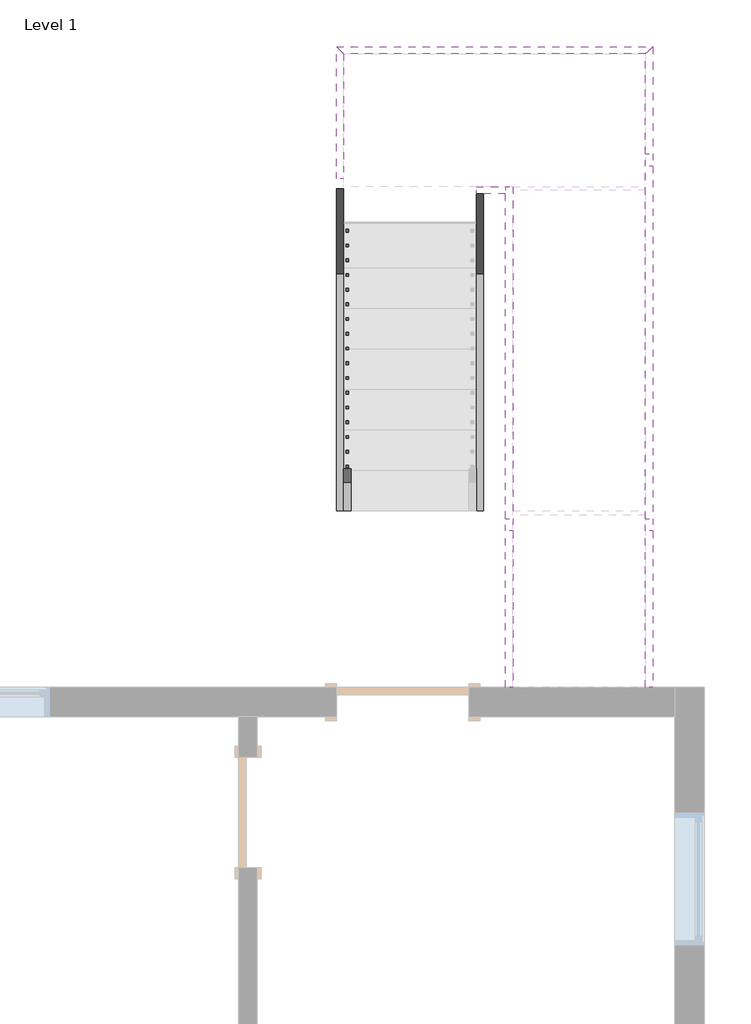
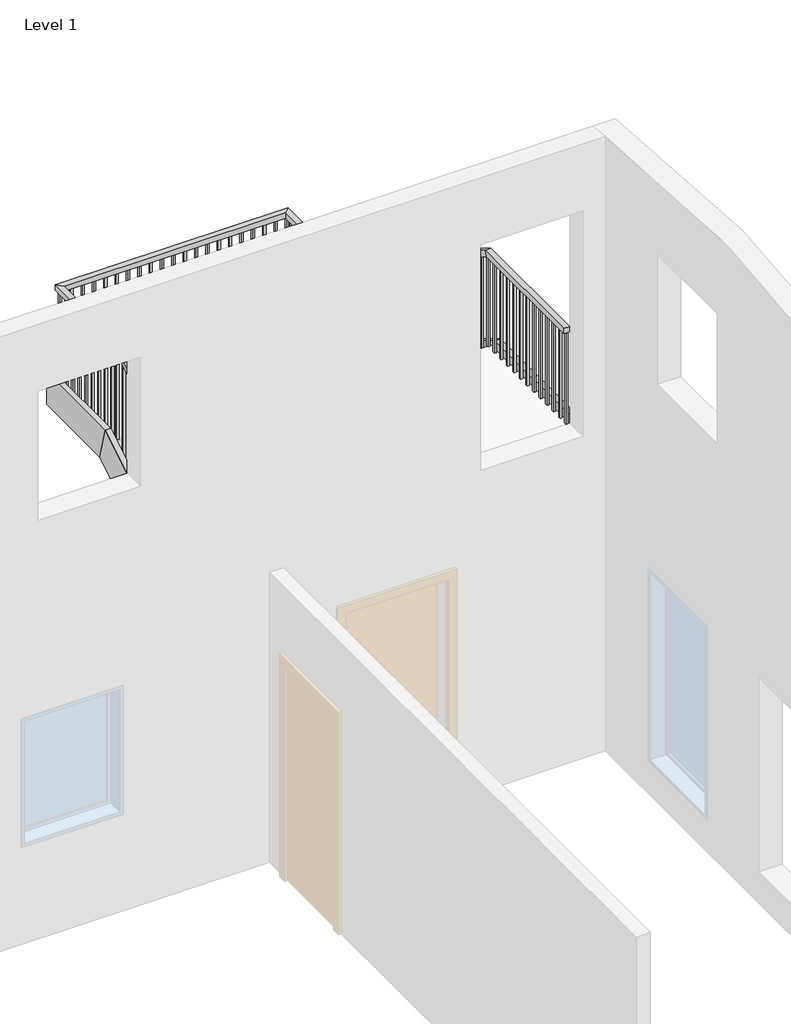
# One storey, part 3 of 3: 10 members, 1 railing.
"""IFC4 building model written with IfcOpenShell, lengths in millimetres."""

from ifc_helpers import new_model, si_unit, frame, origin, place, context, project, spatial, polyline, outline, extrude, faceted_brep, element, save

model = new_model("IFC4")

# Units and contexts
model_context = context("Model", 3, world=origin())
ifc_project = project(units=[si_unit("LENGTHUNIT", "METRE", prefix="MILLI")], contexts=[model_context])

# Site, building, storey
site = spatial("IfcSite", under=ifc_project)
building = spatial("IfcBuilding", under=site)
storey = spatial("IfcBuildingStorey", under=building, Name="Level 1", Elevation=0.0)

# Members
placement = place(None, origin())
element("IfcMember", 1, ObjectType="Stringer - 2\" Width", at=placement, inside=storey, context=model_context, shape_type="SweptSolid", body=[
    extrude(outline(polyline([(14886.0483822, 0.0), (14886.0483822, 212.114512), (17176.3894375, 1600.2), (17261.543894, 1295.4), (15124.133894, 0.0), (14886.0483822, 0.0)])), frame((14862.3123343, 0.0, 0.0), z_axis=(1.0, 0.0, 0.0), x_axis=(0.0, 1.0, 0.0)), (0.0, 0.0, 1.0), 50.8),
])
element("IfcMember", 2, ObjectType="Stringer - 2\" Width", at=placement, inside=storey, context=model_context, shape_type="SweptSolid", body=[
    extrude(outline(polyline([(14886.0483822, 0.0), (14886.0483822, 212.114512), (17070.4483822, 1535.9932998), (17070.4483822, 1179.5845383), (15124.133894, 0.0), (14886.0483822, 0.0)])), frame((15827.5123343, 0.0, 0.0), z_axis=(1.0, 0.0, 0.0), x_axis=(0.0, 1.0, 0.0)), (0.0, 0.0, 1.0), 50.8),
])
element("IfcMember", 3, ObjectType="Stringer - 2\" Width", at=placement, inside=storey, context=model_context, shape_type="SweptSolid", body=[
    extrude(outline(polyline([(17345.507327, 1600.2), (17260.3528705, 1295.4), (14745.7528705, 2819.4), (14830.907327, 3124.2), (17345.507327, 1600.2)])), frame((16995.9123343, 0.0, 0.0), z_axis=(1.0, 0.0, 0.0), x_axis=(0.0, 1.0, 0.0)), (0.0, 0.0, 1.0), 50.8),
])
element("IfcMember", 4, ObjectType="Stringer - 2\" Width", at=placement, inside=storey, context=model_context, shape_type="SweptSolid", body=[
    extrude(outline(polyline([(17121.2483822, 1736.114512), (17121.2483822, 1379.7057504), (14745.7528705, 2819.4), (14830.907327, 3124.2), (17121.2483822, 1736.114512)])), frame((16030.7123343, 0.0, 0.0), z_axis=(1.0, 0.0, 0.0), x_axis=(0.0, 1.0, 0.0)), (0.0, 0.0, 1.0), 50.8),
])
element("IfcMember", 5, ObjectType="Stringer - 2\" Width", at=placement, inside=storey, context=model_context, shape_type="Brep", body=[
    faceted_brep([(16995.9123343, 17345.507327, 1600.2), (17046.7123343, 17345.507327, 1600.2), (17046.7123343, 18086.4483822, 1600.2), (16995.9123343, 18035.6483822, 1600.2), (16995.9123343, 17260.3528705, 1295.4), (16995.9123343, 18035.6483822, 1295.4), (17046.7123343, 17260.3528705, 1295.4), (17046.7123343, 18086.4483822, 1295.4)], [[[0, 1, 2, 3]], [[4, 0, 3, 5]], [[6, 4, 5, 7]], [[1, 6, 7, 2]], [[1, 0, 4, 6]], [[2, 7, 5, 3]]]),
])
element("IfcMember", 6, ObjectType="Stringer - 2\" Width", at=placement, inside=storey, context=model_context, shape_type="SweptSolid", body=[
    extrude(outline(polyline([(17046.7123343, 18086.4483822), (16995.9123343, 18035.6483822), (14913.1123343, 18035.6483822), (14862.3123343, 18086.4483822), (17046.7123343, 18086.4483822)])), frame((0.0, 0.0, 1295.4), z_axis=(0.0, 0.0, 1.0), x_axis=(1.0, 0.0, 0.0)), (0.0, 0.0, 1.0), 304.8),
])
element("IfcMember", 7, ObjectType="Stringer - 2\" Width", at=placement, inside=storey, context=model_context, shape_type="Brep", body=[
    faceted_brep([(14913.1123343, 18035.6483822, 1600.2), (14862.3123343, 18086.4483822, 1600.2), (14862.3123343, 17176.3894375, 1600.2), (14913.1123343, 17176.3894375, 1600.2), (14913.1123343, 18035.6483822, 1295.4), (14913.1123343, 17261.543894, 1295.4), (14862.3123343, 18086.4483822, 1295.4), (14862.3123343, 17261.543894, 1295.4)], [[[0, 1, 2, 3]], [[4, 0, 3, 5]], [[6, 4, 5, 7]], [[1, 6, 7, 2]], [[1, 0, 4, 6]], [[2, 7, 5, 3]]]),
])
element("IfcMember", 8, ObjectType="Stringer - 2\" Width", at=placement, inside=storey, context=model_context, shape_type="SweptSolid", body=[
    extrude(outline(polyline([(15827.5123343, 17070.4483822), (15827.5123343, 17121.2483822), (16030.7123343, 17121.2483822), (16030.7123343, 17070.4483822), (15827.5123343, 17070.4483822)])), frame((0.0, 0.0, 1295.4), z_axis=(0.0, 0.0, 1.0), x_axis=(1.0, 0.0, 0.0)), (0.0, 0.0, 1.0), 304.8),
])
element("IfcMember", 9, ObjectType="Stringer - 2\" Width", at=placement, inside=storey, context=model_context, shape_type="SweptSolid", body=[
    extrude(outline(polyline([(13666.8483822, 2819.4), (13666.8483822, 3124.2), (14830.907327, 3124.2), (14745.7528705, 2819.4), (13666.8483822, 2819.4)])), frame((16995.9123343, 0.0, 0.0), z_axis=(1.0, 0.0, 0.0), x_axis=(0.0, 1.0, 0.0)), (0.0, 0.0, 1.0), 50.8),
])
element("IfcMember", 10, ObjectType="Stringer - 2\" Width", at=placement, inside=storey, context=model_context, shape_type="SweptSolid", body=[
    extrude(outline(polyline([(14830.907327, 3124.2), (14745.7528705, 2819.4), (13666.8483822, 2819.4), (13666.8483822, 3124.2), (14830.907327, 3124.2)])), frame((16030.7123343, 0.0, 0.0), z_axis=(1.0, 0.0, 0.0), x_axis=(0.0, 1.0, 0.0)), (0.0, 0.0, 1.0), 50.8),
])

# Railing
element("IfcRailing", 11, ObjectType="Handrail - Rectangular", at=placement, inside=storey, context=model_context, shape_type="SolidModel", body=[
    faceted_brep([(16995.9123343, 13666.8483822, 3962.4), (16945.1123343, 13666.8483822, 3962.4), (16945.1123343, 13666.8483822, 3911.6), (16995.9123343, 13666.8483822, 3911.6), (16995.9123343, 14871.8559728, 3911.6), (16995.9123343, 14886.0483822, 3962.4), (16945.1123343, 14871.8559728, 3911.6), (16945.1123343, 14886.0483822, 3962.4), (16995.9123343, 17094.918655, 2564.2892835), (16995.9123343, 17121.2483822, 2607.7333333), (16945.1123343, 17094.918655, 2564.2892835), (16945.1123343, 17121.2483822, 2607.7333333), (16995.9123343, 17386.4559728, 2387.6), (16995.9123343, 17400.6483822, 2438.4), (16945.1123343, 17386.4559728, 2387.6), (16945.1123343, 17400.6483822, 2438.4), (14913.1123343, 18035.6483822, 2387.6), (14913.1123343, 18035.6483822, 2438.4), (16995.9123343, 18035.6483822, 2438.4), (16995.9123343, 18035.6483822, 2387.6), (14963.9123343, 17984.8483822, 2387.6), (16945.1123343, 17984.8483822, 2387.6), (14963.9123343, 17984.8483822, 2438.4), (16945.1123343, 17984.8483822, 2438.4), (14913.1123343, 17135.4407916, 2387.6), (14913.1123343, 17121.2483822, 2438.4), (14963.9123343, 17135.4407916, 2387.6), (14963.9123343, 17121.2483822, 2438.4), (14913.1123343, 14886.0483822, 1083.7333333), (14913.1123343, 14886.0483822, 1024.3318731), (14963.9123343, 14886.0483822, 1024.3318731), (14963.9123343, 14886.0483822, 1083.7333333)], [[[0, 1, 2, 3]], [[4, 5, 0, 3]], [[6, 4, 3, 2]], [[7, 6, 2, 1]], [[5, 7, 1, 0]], [[8, 9, 5, 4]], [[10, 8, 4, 6]], [[11, 10, 6, 7]], [[9, 11, 7, 5]], [[12, 13, 9, 8]], [[14, 12, 8, 10]], [[15, 14, 10, 11]], [[13, 15, 11, 9]], [[16, 17, 18, 19]], [[20, 16, 19, 21]], [[22, 20, 21, 23]], [[17, 22, 23, 18]], [[24, 25, 17, 16]], [[26, 24, 16, 20]], [[27, 26, 20, 22]], [[25, 27, 22, 17]], [[28, 29, 30, 31]], [[29, 28, 25, 24]], [[30, 29, 24, 26]], [[31, 30, 26, 27]], [[28, 31, 27, 25]], [[19, 18, 13, 12]], [[21, 19, 12, 14]], [[23, 21, 14, 15]], [[18, 23, 15, 13]]]),
    extrude(outline(polyline([(14978.1233822, 1080.1349034), (14997.1733822, 1091.6803579), (14997.1733822, 169.3333333), (14978.1233822, 169.3333333), (14978.1233822, 1080.1349034)])), frame((14928.9873343, 0.0, 0.0), z_axis=(1.0, 0.0, 0.0), x_axis=(0.0, 1.0, 0.0)), (0.0, 0.0, 1.0), 19.05),
    extrude(outline(polyline([(15079.7233822, 1141.710661), (15098.7733822, 1153.2561155), (15098.7733822, 169.3333333), (15079.7233822, 169.3333333), (15079.7233822, 1141.710661)])), frame((14928.9873343, 0.0, 0.0), z_axis=(1.0, 0.0, 0.0), x_axis=(0.0, 1.0, 0.0)), (0.0, 0.0, 1.0), 19.05),
    extrude(outline(polyline([(15181.3233822, 1203.2864185), (15200.3733822, 1214.8318731), (15200.3733822, 338.6666667), (15181.3233822, 338.6666667), (15181.3233822, 1203.2864185)])), frame((14928.9873343, 0.0, 0.0), z_axis=(1.0, 0.0, 0.0), x_axis=(0.0, 1.0, 0.0)), (0.0, 0.0, 1.0), 19.05),
    extrude(outline(polyline([(15282.9233822, 1264.8621761), (15301.9733822, 1276.4076307), (15301.9733822, 338.6666667), (15282.9233822, 338.6666667), (15282.9233822, 1264.8621761)])), frame((14928.9873343, 0.0, 0.0), z_axis=(1.0, 0.0, 0.0), x_axis=(0.0, 1.0, 0.0)), (0.0, 0.0, 1.0), 19.05),
    extrude(outline(polyline([(15384.5233822, 1326.4379337), (15403.5733822, 1337.9833882), (15403.5733822, 338.6666667), (15384.5233822, 338.6666667), (15384.5233822, 1326.4379337)])), frame((14928.9873343, 0.0, 0.0), z_axis=(1.0, 0.0, 0.0), x_axis=(0.0, 1.0, 0.0)), (0.0, 0.0, 1.0), 19.05),
    extrude(outline(polyline([(15486.1233822, 1388.0136913), (15505.1733822, 1399.5591458), (15505.1733822, 508.0), (15486.1233822, 508.0), (15486.1233822, 1388.0136913)])), frame((14928.9873343, 0.0, 0.0), z_axis=(1.0, 0.0, 0.0), x_axis=(0.0, 1.0, 0.0)), (0.0, 0.0, 1.0), 19.05),
    extrude(outline(polyline([(15587.7233822, 1449.5894488), (15606.7733822, 1461.1349034), (15606.7733822, 508.0), (15587.7233822, 508.0), (15587.7233822, 1449.5894488)])), frame((14928.9873343, 0.0, 0.0), z_axis=(1.0, 0.0, 0.0), x_axis=(0.0, 1.0, 0.0)), (0.0, 0.0, 1.0), 19.05),
    extrude(outline(polyline([(15689.3233822, 1511.1652064), (15708.3733822, 1522.710661), (15708.3733822, 508.0), (15689.3233822, 508.0), (15689.3233822, 1511.1652064)])), frame((14928.9873343, 0.0, 0.0), z_axis=(1.0, 0.0, 0.0), x_axis=(0.0, 1.0, 0.0)), (0.0, 0.0, 1.0), 19.05),
    extrude(outline(polyline([(15790.9233822, 1572.740964), (15809.9733822, 1584.2864185), (15809.9733822, 677.3333333), (15790.9233822, 677.3333333), (15790.9233822, 1572.740964)])), frame((14928.9873343, 0.0, 0.0), z_axis=(1.0, 0.0, 0.0), x_axis=(0.0, 1.0, 0.0)), (0.0, 0.0, 1.0), 19.05),
    extrude(outline(polyline([(15892.5233822, 1634.3167216), (15911.5733822, 1645.8621761), (15911.5733822, 677.3333333), (15892.5233822, 677.3333333), (15892.5233822, 1634.3167216)])), frame((14928.9873343, 0.0, 0.0), z_axis=(1.0, 0.0, 0.0), x_axis=(0.0, 1.0, 0.0)), (0.0, 0.0, 1.0), 19.05),
    extrude(outline(polyline([(15994.1233822, 1695.8924791), (16013.1733822, 1707.4379337), (16013.1733822, 846.6666667), (15994.1233822, 846.6666667), (15994.1233822, 1695.8924791)])), frame((14928.9873343, 0.0, 0.0), z_axis=(1.0, 0.0, 0.0), x_axis=(0.0, 1.0, 0.0)), (0.0, 0.0, 1.0), 19.05),
    extrude(outline(polyline([(16095.7233822, 1757.4682367), (16114.7733822, 1769.0136913), (16114.7733822, 846.6666667), (16095.7233822, 846.6666667), (16095.7233822, 1757.4682367)])), frame((14928.9873343, 0.0, 0.0), z_axis=(1.0, 0.0, 0.0), x_axis=(0.0, 1.0, 0.0)), (0.0, 0.0, 1.0), 19.05),
    extrude(outline(polyline([(16197.3233822, 1819.0439943), (16216.3733822, 1830.5894488), (16216.3733822, 846.6666667), (16197.3233822, 846.6666667), (16197.3233822, 1819.0439943)])), frame((14928.9873343, 0.0, 0.0), z_axis=(1.0, 0.0, 0.0), x_axis=(0.0, 1.0, 0.0)), (0.0, 0.0, 1.0), 19.05),
    extrude(outline(polyline([(16298.9233822, 1880.6197519), (16317.9733822, 1892.1652064), (16317.9733822, 1016.0), (16298.9233822, 1016.0), (16298.9233822, 1880.6197519)])), frame((14928.9873343, 0.0, 0.0), z_axis=(1.0, 0.0, 0.0), x_axis=(0.0, 1.0, 0.0)), (0.0, 0.0, 1.0), 19.05),
    extrude(outline(polyline([(16400.5233822, 1942.1955094), (16419.5733822, 1953.740964), (16419.5733822, 1016.0), (16400.5233822, 1016.0), (16400.5233822, 1942.1955094)])), frame((14928.9873343, 0.0, 0.0), z_axis=(1.0, 0.0, 0.0), x_axis=(0.0, 1.0, 0.0)), (0.0, 0.0, 1.0), 19.05),
    extrude(outline(polyline([(16502.1233822, 2003.771267), (16521.1733822, 2015.3167216), (16521.1733822, 1016.0), (16502.1233822, 1016.0), (16502.1233822, 2003.771267)])), frame((14928.9873343, 0.0, 0.0), z_axis=(1.0, 0.0, 0.0), x_axis=(0.0, 1.0, 0.0)), (0.0, 0.0, 1.0), 19.05),
    extrude(outline(polyline([(16603.7233822, 2065.3470246), (16622.7733822, 2076.8924791), (16622.7733822, 1185.3333333), (16603.7233822, 1185.3333333), (16603.7233822, 2065.3470246)])), frame((14928.9873343, 0.0, 0.0), z_axis=(1.0, 0.0, 0.0), x_axis=(0.0, 1.0, 0.0)), (0.0, 0.0, 1.0), 19.05),
    extrude(outline(polyline([(16705.3233822, 2126.9227822), (16724.3733822, 2138.4682367), (16724.3733822, 1185.3333333), (16705.3233822, 1185.3333333), (16705.3233822, 2126.9227822)])), frame((14928.9873343, 0.0, 0.0), z_axis=(1.0, 0.0, 0.0), x_axis=(0.0, 1.0, 0.0)), (0.0, 0.0, 1.0), 19.05),
    extrude(outline(polyline([(16806.9233822, 2188.4985397), (16825.9733822, 2200.0439943), (16825.9733822, 1185.3333333), (16806.9233822, 1185.3333333), (16806.9233822, 2188.4985397)])), frame((14928.9873343, 0.0, 0.0), z_axis=(1.0, 0.0, 0.0), x_axis=(0.0, 1.0, 0.0)), (0.0, 0.0, 1.0), 19.05),
    extrude(outline(polyline([(16908.5233822, 2250.0742973), (16927.5733822, 2261.6197519), (16927.5733822, 1354.6666667), (16908.5233822, 1354.6666667), (16908.5233822, 2250.0742973)])), frame((14928.9873343, 0.0, 0.0), z_axis=(1.0, 0.0, 0.0), x_axis=(0.0, 1.0, 0.0)), (0.0, 0.0, 1.0), 19.05),
    extrude(outline(polyline([(17010.1233822, 2311.6500549), (17029.1733822, 2323.1955094), (17029.1733822, 1354.6666667), (17010.1233822, 1354.6666667), (17010.1233822, 2311.6500549)])), frame((14928.9873343, 0.0, 0.0), z_axis=(1.0, 0.0, 0.0), x_axis=(0.0, 1.0, 0.0)), (0.0, 0.0, 1.0), 19.05),
    extrude(outline(polyline([(14928.9873343, 17206.9733822), (14948.0373343, 17206.9733822), (14948.0373343, 17187.9233822), (14928.9873343, 17187.9233822), (14928.9873343, 17206.9733822)])), frame((0.0, 0.0, 1524.0), z_axis=(0.0, 0.0, 1.0), x_axis=(1.0, 0.0, 0.0)), (0.0, 0.0, 1.0), 863.6),
    extrude(outline(polyline([(14928.9873343, 17308.5733822), (14948.0373343, 17308.5733822), (14948.0373343, 17289.5233822), (14928.9873343, 17289.5233822), (14928.9873343, 17308.5733822)])), frame((0.0, 0.0, 1524.0), z_axis=(0.0, 0.0, 1.0), x_axis=(1.0, 0.0, 0.0)), (0.0, 0.0, 1.0), 863.6),
    extrude(outline(polyline([(14928.9873343, 17410.1733822), (14948.0373343, 17410.1733822), (14948.0373343, 17391.1233822), (14928.9873343, 17391.1233822), (14928.9873343, 17410.1733822)])), frame((0.0, 0.0, 1524.0), z_axis=(0.0, 0.0, 1.0), x_axis=(1.0, 0.0, 0.0)), (0.0, 0.0, 1.0), 863.6),
    extrude(outline(polyline([(14928.9873343, 17511.7733822), (14948.0373343, 17511.7733822), (14948.0373343, 17492.7233822), (14928.9873343, 17492.7233822), (14928.9873343, 17511.7733822)])), frame((0.0, 0.0, 1524.0), z_axis=(0.0, 0.0, 1.0), x_axis=(1.0, 0.0, 0.0)), (0.0, 0.0, 1.0), 863.6),
    extrude(outline(polyline([(14928.9873343, 17613.3733822), (14948.0373343, 17613.3733822), (14948.0373343, 17594.3233822), (14928.9873343, 17594.3233822), (14928.9873343, 17613.3733822)])), frame((0.0, 0.0, 1524.0), z_axis=(0.0, 0.0, 1.0), x_axis=(1.0, 0.0, 0.0)), (0.0, 0.0, 1.0), 863.6),
    extrude(outline(polyline([(14928.9873343, 17714.9733822), (14948.0373343, 17714.9733822), (14948.0373343, 17695.9233822), (14928.9873343, 17695.9233822), (14928.9873343, 17714.9733822)])), frame((0.0, 0.0, 1524.0), z_axis=(0.0, 0.0, 1.0), x_axis=(1.0, 0.0, 0.0)), (0.0, 0.0, 1.0), 863.6),
    extrude(outline(polyline([(14928.9873343, 17816.5733822), (14948.0373343, 17816.5733822), (14948.0373343, 17797.5233822), (14928.9873343, 17797.5233822), (14928.9873343, 17816.5733822)])), frame((0.0, 0.0, 1524.0), z_axis=(0.0, 0.0, 1.0), x_axis=(1.0, 0.0, 0.0)), (0.0, 0.0, 1.0), 863.6),
    extrude(outline(polyline([(14928.9873343, 17918.1733822), (14948.0373343, 17918.1733822), (14948.0373343, 17899.1233822), (14928.9873343, 17899.1233822), (14928.9873343, 17918.1733822)])), frame((0.0, 0.0, 1524.0), z_axis=(0.0, 0.0, 1.0), x_axis=(1.0, 0.0, 0.0)), (0.0, 0.0, 1.0), 863.6),
    extrude(outline(polyline([(15049.6373343, 18019.7733822), (15049.6373343, 18000.7233822), (15030.5873343, 18000.7233822), (15030.5873343, 18019.7733822), (15049.6373343, 18019.7733822)])), frame((0.0, 0.0, 1524.0), z_axis=(0.0, 0.0, 1.0), x_axis=(1.0, 0.0, 0.0)), (0.0, 0.0, 1.0), 863.6),
    extrude(outline(polyline([(15151.2373343, 18019.7733822), (15151.2373343, 18000.7233822), (15132.1873343, 18000.7233822), (15132.1873343, 18019.7733822), (15151.2373343, 18019.7733822)])), frame((0.0, 0.0, 1524.0), z_axis=(0.0, 0.0, 1.0), x_axis=(1.0, 0.0, 0.0)), (0.0, 0.0, 1.0), 863.6),
    extrude(outline(polyline([(15252.8373343, 18019.7733822), (15252.8373343, 18000.7233822), (15233.7873343, 18000.7233822), (15233.7873343, 18019.7733822), (15252.8373343, 18019.7733822)])), frame((0.0, 0.0, 1524.0), z_axis=(0.0, 0.0, 1.0), x_axis=(1.0, 0.0, 0.0)), (0.0, 0.0, 1.0), 863.6),
    extrude(outline(polyline([(15354.4373343, 18019.7733822), (15354.4373343, 18000.7233822), (15335.3873343, 18000.7233822), (15335.3873343, 18019.7733822), (15354.4373343, 18019.7733822)])), frame((0.0, 0.0, 1524.0), z_axis=(0.0, 0.0, 1.0), x_axis=(1.0, 0.0, 0.0)), (0.0, 0.0, 1.0), 863.6),
    extrude(outline(polyline([(15456.0373343, 18019.7733822), (15456.0373343, 18000.7233822), (15436.9873343, 18000.7233822), (15436.9873343, 18019.7733822), (15456.0373343, 18019.7733822)])), frame((0.0, 0.0, 1524.0), z_axis=(0.0, 0.0, 1.0), x_axis=(1.0, 0.0, 0.0)), (0.0, 0.0, 1.0), 863.6),
    extrude(outline(polyline([(15557.6373343, 18019.7733822), (15557.6373343, 18000.7233822), (15538.5873343, 18000.7233822), (15538.5873343, 18019.7733822), (15557.6373343, 18019.7733822)])), frame((0.0, 0.0, 1524.0), z_axis=(0.0, 0.0, 1.0), x_axis=(1.0, 0.0, 0.0)), (0.0, 0.0, 1.0), 863.6),
    extrude(outline(polyline([(15659.2373343, 18019.7733822), (15659.2373343, 18000.7233822), (15640.1873343, 18000.7233822), (15640.1873343, 18019.7733822), (15659.2373343, 18019.7733822)])), frame((0.0, 0.0, 1524.0), z_axis=(0.0, 0.0, 1.0), x_axis=(1.0, 0.0, 0.0)), (0.0, 0.0, 1.0), 863.6),
    extrude(outline(polyline([(15760.8373343, 18019.7733822), (15760.8373343, 18000.7233822), (15741.7873343, 18000.7233822), (15741.7873343, 18019.7733822), (15760.8373343, 18019.7733822)])), frame((0.0, 0.0, 1524.0), z_axis=(0.0, 0.0, 1.0), x_axis=(1.0, 0.0, 0.0)), (0.0, 0.0, 1.0), 863.6),
    extrude(outline(polyline([(15862.4373343, 18019.7733822), (15862.4373343, 18000.7233822), (15843.3873343, 18000.7233822), (15843.3873343, 18019.7733822), (15862.4373343, 18019.7733822)])), frame((0.0, 0.0, 1524.0), z_axis=(0.0, 0.0, 1.0), x_axis=(1.0, 0.0, 0.0)), (0.0, 0.0, 1.0), 863.6),
    extrude(outline(polyline([(15964.0373343, 18019.7733822), (15964.0373343, 18000.7233822), (15944.9873343, 18000.7233822), (15944.9873343, 18019.7733822), (15964.0373343, 18019.7733822)])), frame((0.0, 0.0, 1524.0), z_axis=(0.0, 0.0, 1.0), x_axis=(1.0, 0.0, 0.0)), (0.0, 0.0, 1.0), 863.6),
    extrude(outline(polyline([(16065.6373343, 18019.7733822), (16065.6373343, 18000.7233822), (16046.5873343, 18000.7233822), (16046.5873343, 18019.7733822), (16065.6373343, 18019.7733822)])), frame((0.0, 0.0, 1524.0), z_axis=(0.0, 0.0, 1.0), x_axis=(1.0, 0.0, 0.0)), (0.0, 0.0, 1.0), 863.6),
    extrude(outline(polyline([(16167.2373343, 18019.7733822), (16167.2373343, 18000.7233822), (16148.1873343, 18000.7233822), (16148.1873343, 18019.7733822), (16167.2373343, 18019.7733822)])), frame((0.0, 0.0, 1524.0), z_axis=(0.0, 0.0, 1.0), x_axis=(1.0, 0.0, 0.0)), (0.0, 0.0, 1.0), 863.6),
    extrude(outline(polyline([(16268.8373343, 18019.7733822), (16268.8373343, 18000.7233822), (16249.7873343, 18000.7233822), (16249.7873343, 18019.7733822), (16268.8373343, 18019.7733822)])), frame((0.0, 0.0, 1524.0), z_axis=(0.0, 0.0, 1.0), x_axis=(1.0, 0.0, 0.0)), (0.0, 0.0, 1.0), 863.6),
    extrude(outline(polyline([(16370.4373343, 18019.7733822), (16370.4373343, 18000.7233822), (16351.3873343, 18000.7233822), (16351.3873343, 18019.7733822), (16370.4373343, 18019.7733822)])), frame((0.0, 0.0, 1524.0), z_axis=(0.0, 0.0, 1.0), x_axis=(1.0, 0.0, 0.0)), (0.0, 0.0, 1.0), 863.6),
    extrude(outline(polyline([(16472.0373343, 18019.7733822), (16472.0373343, 18000.7233822), (16452.9873343, 18000.7233822), (16452.9873343, 18019.7733822), (16472.0373343, 18019.7733822)])), frame((0.0, 0.0, 1524.0), z_axis=(0.0, 0.0, 1.0), x_axis=(1.0, 0.0, 0.0)), (0.0, 0.0, 1.0), 863.6),
    extrude(outline(polyline([(16573.6373343, 18019.7733822), (16573.6373343, 18000.7233822), (16554.5873343, 18000.7233822), (16554.5873343, 18019.7733822), (16573.6373343, 18019.7733822)])), frame((0.0, 0.0, 1524.0), z_axis=(0.0, 0.0, 1.0), x_axis=(1.0, 0.0, 0.0)), (0.0, 0.0, 1.0), 863.6),
    extrude(outline(polyline([(16675.2373343, 18019.7733822), (16675.2373343, 18000.7233822), (16656.1873343, 18000.7233822), (16656.1873343, 18019.7733822), (16675.2373343, 18019.7733822)])), frame((0.0, 0.0, 1524.0), z_axis=(0.0, 0.0, 1.0), x_axis=(1.0, 0.0, 0.0)), (0.0, 0.0, 1.0), 863.6),
    extrude(outline(polyline([(16776.8373343, 18019.7733822), (16776.8373343, 18000.7233822), (16757.7873343, 18000.7233822), (16757.7873343, 18019.7733822), (16776.8373343, 18019.7733822)])), frame((0.0, 0.0, 1524.0), z_axis=(0.0, 0.0, 1.0), x_axis=(1.0, 0.0, 0.0)), (0.0, 0.0, 1.0), 863.6),
    extrude(outline(polyline([(16878.4373343, 18019.7733822), (16878.4373343, 18000.7233822), (16859.3873343, 18000.7233822), (16859.3873343, 18019.7733822), (16878.4373343, 18019.7733822)])), frame((0.0, 0.0, 1524.0), z_axis=(0.0, 0.0, 1.0), x_axis=(1.0, 0.0, 0.0)), (0.0, 0.0, 1.0), 863.6),
    extrude(outline(polyline([(16980.0373343, 17924.5233822), (16960.9873343, 17924.5233822), (16960.9873343, 17943.5733822), (16980.0373343, 17943.5733822), (16980.0373343, 17924.5233822)])), frame((0.0, 0.0, 1524.0), z_axis=(0.0, 0.0, 1.0), x_axis=(1.0, 0.0, 0.0)), (0.0, 0.0, 1.0), 863.6),
    extrude(outline(polyline([(16980.0373343, 17822.9233822), (16960.9873343, 17822.9233822), (16960.9873343, 17841.9733822), (16980.0373343, 17841.9733822), (16980.0373343, 17822.9233822)])), frame((0.0, 0.0, 1524.0), z_axis=(0.0, 0.0, 1.0), x_axis=(1.0, 0.0, 0.0)), (0.0, 0.0, 1.0), 863.6),
    extrude(outline(polyline([(16980.0373343, 17721.3233822), (16960.9873343, 17721.3233822), (16960.9873343, 17740.3733822), (16980.0373343, 17740.3733822), (16980.0373343, 17721.3233822)])), frame((0.0, 0.0, 1524.0), z_axis=(0.0, 0.0, 1.0), x_axis=(1.0, 0.0, 0.0)), (0.0, 0.0, 1.0), 863.6),
    extrude(outline(polyline([(16980.0373343, 17619.7233822), (16960.9873343, 17619.7233822), (16960.9873343, 17638.7733822), (16980.0373343, 17638.7733822), (16980.0373343, 17619.7233822)])), frame((0.0, 0.0, 1524.0), z_axis=(0.0, 0.0, 1.0), x_axis=(1.0, 0.0, 0.0)), (0.0, 0.0, 1.0), 863.6),
    extrude(outline(polyline([(16980.0373343, 17518.1233822), (16960.9873343, 17518.1233822), (16960.9873343, 17537.1733822), (16980.0373343, 17537.1733822), (16980.0373343, 17518.1233822)])), frame((0.0, 0.0, 1524.0), z_axis=(0.0, 0.0, 1.0), x_axis=(1.0, 0.0, 0.0)), (0.0, 0.0, 1.0), 863.6),
    extrude(outline(polyline([(16980.0373343, 17416.5233822), (16960.9873343, 17416.5233822), (16960.9873343, 17435.5733822), (16980.0373343, 17435.5733822), (16980.0373343, 17416.5233822)])), frame((0.0, 0.0, 1524.0), z_axis=(0.0, 0.0, 1.0), x_axis=(1.0, 0.0, 0.0)), (0.0, 0.0, 1.0), 863.6),
    extrude(outline(polyline([(17314.9233822, 2430.9530852), (17333.9733822, 2419.4076307), (17333.9733822, 1524.0), (17314.9233822, 1524.0), (17314.9233822, 2430.9530852)])), frame((16960.9873343, 0.0, 0.0), z_axis=(1.0, 0.0, 0.0), x_axis=(0.0, 1.0, 0.0)), (0.0, 0.0, 1.0), 19.05),
    extrude(outline(polyline([(17213.3233822, 2492.5288428), (17232.3733822, 2480.9833882), (17232.3733822, 1524.0), (17213.3233822, 1524.0), (17213.3233822, 2492.5288428)])), frame((16960.9873343, 0.0, 0.0), z_axis=(1.0, 0.0, 0.0), x_axis=(0.0, 1.0, 0.0)), (0.0, 0.0, 1.0), 19.05),
    extrude(outline(polyline([(17010.1233822, 2615.6803579), (17029.1733822, 2604.1349034), (17029.1733822, 1693.3333333), (17010.1233822, 1693.3333333), (17010.1233822, 2615.6803579)])), frame((16960.9873343, 0.0, 0.0), z_axis=(1.0, 0.0, 0.0), x_axis=(0.0, 1.0, 0.0)), (0.0, 0.0, 1.0), 19.05),
    extrude(outline(polyline([(16908.5233822, 2677.2561155), (16927.5733822, 2665.710661), (16927.5733822, 1693.3333333), (16908.5233822, 1693.3333333), (16908.5233822, 2677.2561155)])), frame((16960.9873343, 0.0, 0.0), z_axis=(1.0, 0.0, 0.0), x_axis=(0.0, 1.0, 0.0)), (0.0, 0.0, 1.0), 19.05),
    extrude(outline(polyline([(16806.9233822, 2738.8318731), (16825.9733822, 2727.2864185), (16825.9733822, 1862.6666667), (16806.9233822, 1862.6666667), (16806.9233822, 2738.8318731)])), frame((16960.9873343, 0.0, 0.0), z_axis=(1.0, 0.0, 0.0), x_axis=(0.0, 1.0, 0.0)), (0.0, 0.0, 1.0), 19.05),
    extrude(outline(polyline([(16705.3233822, 2800.4076307), (16724.3733822, 2788.8621761), (16724.3733822, 1862.6666667), (16705.3233822, 1862.6666667), (16705.3233822, 2800.4076307)])), frame((16960.9873343, 0.0, 0.0), z_axis=(1.0, 0.0, 0.0), x_axis=(0.0, 1.0, 0.0)), (0.0, 0.0, 1.0), 19.05),
    extrude(outline(polyline([(16603.7233822, 2861.9833882), (16622.7733822, 2850.4379337), (16622.7733822, 1862.6666667), (16603.7233822, 1862.6666667), (16603.7233822, 2861.9833882)])), frame((16960.9873343, 0.0, 0.0), z_axis=(1.0, 0.0, 0.0), x_axis=(0.0, 1.0, 0.0)), (0.0, 0.0, 1.0), 19.05),
    extrude(outline(polyline([(16502.1233822, 2923.5591458), (16521.1733822, 2912.0136913), (16521.1733822, 2032.0), (16502.1233822, 2032.0), (16502.1233822, 2923.5591458)])), frame((16960.9873343, 0.0, 0.0), z_axis=(1.0, 0.0, 0.0), x_axis=(0.0, 1.0, 0.0)), (0.0, 0.0, 1.0), 19.05),
    extrude(outline(polyline([(16400.5233822, 2985.1349034), (16419.5733822, 2973.5894488), (16419.5733822, 2032.0), (16400.5233822, 2032.0), (16400.5233822, 2985.1349034)])), frame((16960.9873343, 0.0, 0.0), z_axis=(1.0, 0.0, 0.0), x_axis=(0.0, 1.0, 0.0)), (0.0, 0.0, 1.0), 19.05),
    extrude(outline(polyline([(16298.9233822, 3046.710661), (16317.9733822, 3035.1652064), (16317.9733822, 2032.0), (16298.9233822, 2032.0), (16298.9233822, 3046.710661)])), frame((16960.9873343, 0.0, 0.0), z_axis=(1.0, 0.0, 0.0), x_axis=(0.0, 1.0, 0.0)), (0.0, 0.0, 1.0), 19.05),
    extrude(outline(polyline([(16197.3233822, 3108.2864185), (16216.3733822, 3096.740964), (16216.3733822, 2201.3333333), (16197.3233822, 2201.3333333), (16197.3233822, 3108.2864185)])), frame((16960.9873343, 0.0, 0.0), z_axis=(1.0, 0.0, 0.0), x_axis=(0.0, 1.0, 0.0)), (0.0, 0.0, 1.0), 19.05),
    extrude(outline(polyline([(16095.7233822, 3169.8621761), (16114.7733822, 3158.3167216), (16114.7733822, 2201.3333333), (16095.7233822, 2201.3333333), (16095.7233822, 3169.8621761)])), frame((16960.9873343, 0.0, 0.0), z_axis=(1.0, 0.0, 0.0), x_axis=(0.0, 1.0, 0.0)), (0.0, 0.0, 1.0), 19.05),
    extrude(outline(polyline([(15994.1233822, 3231.4379337), (16013.1733822, 3219.8924791), (16013.1733822, 2370.6666667), (15994.1233822, 2370.6666667), (15994.1233822, 3231.4379337)])), frame((16960.9873343, 0.0, 0.0), z_axis=(1.0, 0.0, 0.0), x_axis=(0.0, 1.0, 0.0)), (0.0, 0.0, 1.0), 19.05),
    extrude(outline(polyline([(15892.5233822, 3293.0136913), (15911.5733822, 3281.4682367), (15911.5733822, 2370.6666667), (15892.5233822, 2370.6666667), (15892.5233822, 3293.0136913)])), frame((16960.9873343, 0.0, 0.0), z_axis=(1.0, 0.0, 0.0), x_axis=(0.0, 1.0, 0.0)), (0.0, 0.0, 1.0), 19.05),
    extrude(outline(polyline([(15790.9233822, 3354.5894488), (15809.9733822, 3343.0439943), (15809.9733822, 2370.6666667), (15790.9233822, 2370.6666667), (15790.9233822, 3354.5894488)])), frame((16960.9873343, 0.0, 0.0), z_axis=(1.0, 0.0, 0.0), x_axis=(0.0, 1.0, 0.0)), (0.0, 0.0, 1.0), 19.05),
    extrude(outline(polyline([(15689.3233822, 3416.1652064), (15708.3733822, 3404.6197519), (15708.3733822, 2540.0), (15689.3233822, 2540.0), (15689.3233822, 3416.1652064)])), frame((16960.9873343, 0.0, 0.0), z_axis=(1.0, 0.0, 0.0), x_axis=(0.0, 1.0, 0.0)), (0.0, 0.0, 1.0), 19.05),
    extrude(outline(polyline([(15587.7233822, 3477.740964), (15606.7733822, 3466.1955094), (15606.7733822, 2540.0), (15587.7233822, 2540.0), (15587.7233822, 3477.740964)])), frame((16960.9873343, 0.0, 0.0), z_axis=(1.0, 0.0, 0.0), x_axis=(0.0, 1.0, 0.0)), (0.0, 0.0, 1.0), 19.05),
    extrude(outline(polyline([(15486.1233822, 3539.3167216), (15505.1733822, 3527.771267), (15505.1733822, 2540.0), (15486.1233822, 2540.0), (15486.1233822, 3539.3167216)])), frame((16960.9873343, 0.0, 0.0), z_axis=(1.0, 0.0, 0.0), x_axis=(0.0, 1.0, 0.0)), (0.0, 0.0, 1.0), 19.05),
    extrude(outline(polyline([(15384.5233822, 3600.8924791), (15403.5733822, 3589.3470246), (15403.5733822, 2709.3333333), (15384.5233822, 2709.3333333), (15384.5233822, 3600.8924791)])), frame((16960.9873343, 0.0, 0.0), z_axis=(1.0, 0.0, 0.0), x_axis=(0.0, 1.0, 0.0)), (0.0, 0.0, 1.0), 19.05),
    extrude(outline(polyline([(15282.9233822, 3662.4682367), (15301.9733822, 3650.9227822), (15301.9733822, 2709.3333333), (15282.9233822, 2709.3333333), (15282.9233822, 3662.4682367)])), frame((16960.9873343, 0.0, 0.0), z_axis=(1.0, 0.0, 0.0), x_axis=(0.0, 1.0, 0.0)), (0.0, 0.0, 1.0), 19.05),
    extrude(outline(polyline([(15181.3233822, 3724.0439943), (15200.3733822, 3712.4985397), (15200.3733822, 2709.3333333), (15181.3233822, 2709.3333333), (15181.3233822, 3724.0439943)])), frame((16960.9873343, 0.0, 0.0), z_axis=(1.0, 0.0, 0.0), x_axis=(0.0, 1.0, 0.0)), (0.0, 0.0, 1.0), 19.05),
    extrude(outline(polyline([(15079.7233822, 3785.6197519), (15098.7733822, 3774.0742973), (15098.7733822, 2878.6666667), (15079.7233822, 2878.6666667), (15079.7233822, 3785.6197519)])), frame((16960.9873343, 0.0, 0.0), z_axis=(1.0, 0.0, 0.0), x_axis=(0.0, 1.0, 0.0)), (0.0, 0.0, 1.0), 19.05),
    extrude(outline(polyline([(14978.1233822, 3847.1955094), (14997.1733822, 3835.6500549), (14997.1733822, 2878.6666667), (14978.1233822, 2878.6666667), (14978.1233822, 3847.1955094)])), frame((16960.9873343, 0.0, 0.0), z_axis=(1.0, 0.0, 0.0), x_axis=(0.0, 1.0, 0.0)), (0.0, 0.0, 1.0), 19.05),
    extrude(outline(polyline([(16980.0373343, 14774.9233822), (16960.9873343, 14774.9233822), (16960.9873343, 14793.9733822), (16980.0373343, 14793.9733822), (16980.0373343, 14774.9233822)])), frame((0.0, 0.0, 3048.0), z_axis=(0.0, 0.0, 1.0), x_axis=(1.0, 0.0, 0.0)), (0.0, 0.0, 1.0), 863.6),
    extrude(outline(polyline([(16980.0373343, 14673.3233822), (16960.9873343, 14673.3233822), (16960.9873343, 14692.3733822), (16980.0373343, 14692.3733822), (16980.0373343, 14673.3233822)])), frame((0.0, 0.0, 3048.0), z_axis=(0.0, 0.0, 1.0), x_axis=(1.0, 0.0, 0.0)), (0.0, 0.0, 1.0), 863.6),
    extrude(outline(polyline([(16980.0373343, 14571.7233822), (16960.9873343, 14571.7233822), (16960.9873343, 14590.7733822), (16980.0373343, 14590.7733822), (16980.0373343, 14571.7233822)])), frame((0.0, 0.0, 3048.0), z_axis=(0.0, 0.0, 1.0), x_axis=(1.0, 0.0, 0.0)), (0.0, 0.0, 1.0), 863.6),
    extrude(outline(polyline([(16980.0373343, 14470.1233822), (16960.9873343, 14470.1233822), (16960.9873343, 14489.1733822), (16980.0373343, 14489.1733822), (16980.0373343, 14470.1233822)])), frame((0.0, 0.0, 3048.0), z_axis=(0.0, 0.0, 1.0), x_axis=(1.0, 0.0, 0.0)), (0.0, 0.0, 1.0), 863.6),
    extrude(outline(polyline([(16980.0373343, 14368.5233822), (16960.9873343, 14368.5233822), (16960.9873343, 14387.5733822), (16980.0373343, 14387.5733822), (16980.0373343, 14368.5233822)])), frame((0.0, 0.0, 3048.0), z_axis=(0.0, 0.0, 1.0), x_axis=(1.0, 0.0, 0.0)), (0.0, 0.0, 1.0), 863.6),
    extrude(outline(polyline([(16980.0373343, 14266.9233822), (16960.9873343, 14266.9233822), (16960.9873343, 14285.9733822), (16980.0373343, 14285.9733822), (16980.0373343, 14266.9233822)])), frame((0.0, 0.0, 3048.0), z_axis=(0.0, 0.0, 1.0), x_axis=(1.0, 0.0, 0.0)), (0.0, 0.0, 1.0), 863.6),
    extrude(outline(polyline([(16980.0373343, 14165.3233822), (16960.9873343, 14165.3233822), (16960.9873343, 14184.3733822), (16980.0373343, 14184.3733822), (16980.0373343, 14165.3233822)])), frame((0.0, 0.0, 3048.0), z_axis=(0.0, 0.0, 1.0), x_axis=(1.0, 0.0, 0.0)), (0.0, 0.0, 1.0), 863.6),
    extrude(outline(polyline([(16980.0373343, 14063.7233822), (16960.9873343, 14063.7233822), (16960.9873343, 14082.7733822), (16980.0373343, 14082.7733822), (16980.0373343, 14063.7233822)])), frame((0.0, 0.0, 3048.0), z_axis=(0.0, 0.0, 1.0), x_axis=(1.0, 0.0, 0.0)), (0.0, 0.0, 1.0), 863.6),
    extrude(outline(polyline([(16980.0373343, 13962.1233822), (16960.9873343, 13962.1233822), (16960.9873343, 13981.1733822), (16980.0373343, 13981.1733822), (16980.0373343, 13962.1233822)])), frame((0.0, 0.0, 3048.0), z_axis=(0.0, 0.0, 1.0), x_axis=(1.0, 0.0, 0.0)), (0.0, 0.0, 1.0), 863.6),
    extrude(outline(polyline([(16980.0373343, 13860.5233822), (16960.9873343, 13860.5233822), (16960.9873343, 13879.5733822), (16980.0373343, 13879.5733822), (16980.0373343, 13860.5233822)])), frame((0.0, 0.0, 3048.0), z_axis=(0.0, 0.0, 1.0), x_axis=(1.0, 0.0, 0.0)), (0.0, 0.0, 1.0), 863.6),
    extrude(outline(polyline([(16980.0373343, 13758.9233822), (16960.9873343, 13758.9233822), (16960.9873343, 13777.9733822), (16980.0373343, 13777.9733822), (16980.0373343, 13758.9233822)])), frame((0.0, 0.0, 3048.0), z_axis=(0.0, 0.0, 1.0), x_axis=(1.0, 0.0, 0.0)), (0.0, 0.0, 1.0), 863.6),
    extrude(outline(polyline([(14928.9873343, 17130.7733822), (14948.0373343, 17130.7733822), (14948.0373343, 17111.7233822), (14928.9873343, 17111.7233822), (14928.9873343, 17130.7733822)])), frame((0.0, 0.0, 1524.0), z_axis=(0.0, 0.0, 1.0), x_axis=(1.0, 0.0, 0.0)), (0.0, 0.0, 1.0), 863.6),
    extrude(outline(polyline([(14948.0373343, 18019.7733822), (14948.0373343, 18000.7233822), (14928.9873343, 18000.7233822), (14928.9873343, 18019.7733822), (14948.0373343, 18019.7733822)])), frame((0.0, 0.0, 1524.0), z_axis=(0.0, 0.0, 1.0), x_axis=(1.0, 0.0, 0.0)), (0.0, 0.0, 1.0), 863.6),
    extrude(outline(polyline([(16980.0373343, 18000.7233822), (16960.9873343, 18000.7233822), (16960.9873343, 18019.7733822), (16980.0373343, 18019.7733822), (16980.0373343, 18000.7233822)])), frame((0.0, 0.0, 1524.0), z_axis=(0.0, 0.0, 1.0), x_axis=(1.0, 0.0, 0.0)), (0.0, 0.0, 1.0), 863.6),
    extrude(outline(polyline([(17111.7233822, 2554.1046004), (17130.7733822, 2542.5591458), (17130.7733822, 1693.3333333), (17111.7233822, 1693.3333333), (17111.7233822, 2554.1046004)])), frame((16960.9873343, 0.0, 0.0), z_axis=(1.0, 0.0, 0.0), x_axis=(0.0, 1.0, 0.0)), (0.0, 0.0, 1.0), 19.05),
    extrude(outline(polyline([(16980.0373343, 14876.5233822), (16960.9873343, 14876.5233822), (16960.9873343, 14895.5733822), (16980.0373343, 14895.5733822), (16980.0373343, 14876.5233822)])), frame((0.0, 0.0, 3048.0), z_axis=(0.0, 0.0, 1.0), x_axis=(1.0, 0.0, 0.0)), (0.0, 0.0, 1.0), 863.6),
    extrude(outline(polyline([(14886.0483822, 1024.3318731), (14905.0983822, 1035.8773276), (14905.0983822, 169.3333333), (14886.0483822, 169.3333333), (14886.0483822, 1024.3318731)])), frame((14928.9873343, 0.0, 0.0), z_axis=(1.0, 0.0, 0.0), x_axis=(0.0, 1.0, 0.0)), (0.0, 0.0, 1.0), 19.05),
    extrude(outline(polyline([(16980.0373343, 13666.8483822), (16960.9873343, 13666.8483822), (16960.9873343, 13685.8983822), (16980.0373343, 13685.8983822), (16980.0373343, 13666.8483822)])), frame((0.0, 0.0, 3048.0), z_axis=(0.0, 0.0, 1.0), x_axis=(1.0, 0.0, 0.0)), (0.0, 0.0, 1.0), 863.6),
])

save(model, "model.ifc")

# Revit data of these elements
# Project information
#   Organization Name = "G3B Press"
#   Organization Description = "Paul F. Aubin Cosulting Services, Inc."
#   Building Name = "Revit Essentials for Architecture"
#   Author = "Paul F. Aubin"
#   Author Website = "https://www.paulaubin.com"
#   Copyright = "Copyright © 2020 Paul F Aubin, all rights reserved"
#   Project Issue Date = "8/1/2020"
#   Project Status = "Schematic Design"
#   Client Name = "Quick Start Overview"
#   Project Address = "568 Grove ST\nAnytown, IL 60000"
#   Project Name = "Pavilion-Complete"
#   Project Number = "2020.01A"
# Type "Handrail - Rectangular"
#   Assembly Code = "C2010400"
#   built-in parameter 1008612 = 0.0416667 (stored number, unit not read)
#   built-in parameter 1008611 = 0.0416667 (stored number, unit not read)
#   built-in parameter 1008609 = 0.333333 (stored number, unit not read)
#   built-in parameter 1008604 = 0.166667 (stored number, unit not read)
#   built-in parameter 1008603 = 0.166667 (stored number, unit not read)
#   Railing Height = 3' - 0"
#   built-in parameter 1008630 = 2
#   built-in parameter 1008610 = 2
#   built-in parameter 1008618 = Baluster - Square : 3/4"
# Elements 1, 2, 3, 4, 5, 6, 7, 8, 9, 10 (IfcMember, "Stringer - 2\" Width")
#   Phase Created = New Construction
# Element 11 (IfcRailing, "Handrail - Rectangular")
#   Phase Created = New Construction
